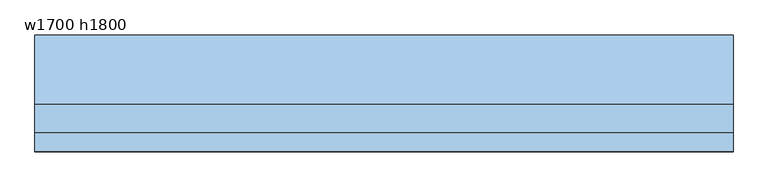
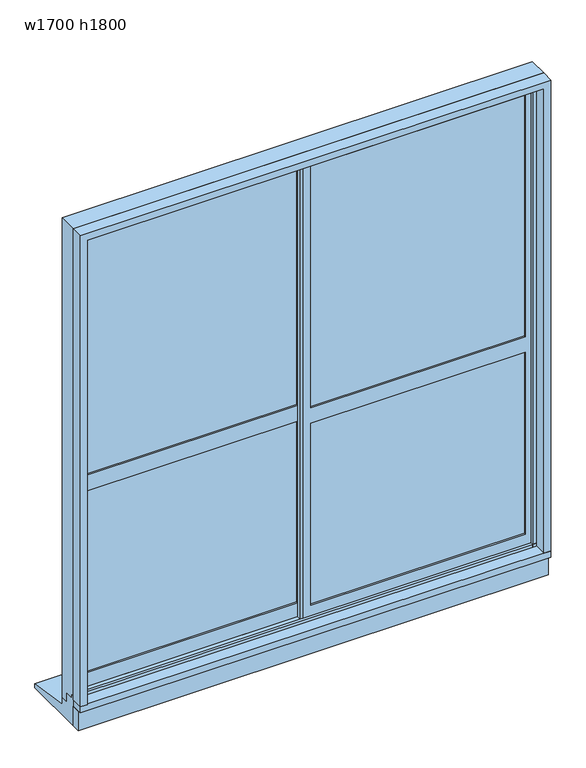
"""IFC4 building model written with IfcOpenShell, lengths in millimetres: window geometry, 引違い窓 2 枚 : w1700 h1800."""

from ifc_helpers import new_model, si_unit, frame, origin, place, context, project, spatial, polyline, outline, extrude, faceted_brep, source, transform, mapped, element, save


def w1700_h1800_203315db(model_context):
    return source(origin(), model_context, "Body", "SolidModel", [
        extrude(outline(polyline([(1860.0, -850.0), (60.0, -850.0), (60.0, -825.0), (1835.0, -825.0), (1835.0, 825.0), (60.0, 825.0), (60.0, 850.0), (1860.0, 850.0), (1860.0, -850.0)])), frame((0.0, -115.0, 0.0), z_axis=(0.0, 1.0, 0.0), x_axis=(0.0, 0.0, 1.0)), (0.0, 0.0, 1.0), 45.0),
        extrude(outline(polyline([(60.0, -850.0), (60.0, -825.0), (1835.0, -825.0), (1835.0, 825.0), (60.0, 825.0), (60.0, 850.0), (1860.0, 850.0), (1860.0, -850.0), (60.0, -850.0)])), frame((0.0, -115.0, 0.0), z_axis=(0.0, 1.0, 0.0), x_axis=(0.0, 0.0, 1.0)), (0.0, 0.0, 1.0), 45.0),
        extrude(outline(polyline([(850.0, -100.0), (-850.0, -100.0), (-850.0, -70.0), (850.0, -70.0), (850.0, -100.0)])), frame((0.0, 0.0, -40.0), z_axis=(0.0, 0.0, 1.0), x_axis=(1.0, 0.0, 0.0)), (0.0, 0.0, 1.0), 75.0),
        extrude(outline(polyline([(15.0, -28.0), (15.0, -42.0), (-15.0, -42.0), (-15.0, -28.0), (15.0, -28.0)])), frame((0.0, 0.0, 60.0), z_axis=(0.0, 0.0, 1.0), x_axis=(1.0, 0.0, 0.0)), (0.0, 0.0, 1.0), 1790.0),
        extrude(outline(polyline([(15.0, -48.5), (790.0, -48.5), (790.0, -53.5), (15.0, -53.5), (15.0, -48.5)])), frame((0.0, 0.0, 867.0), z_axis=(0.0, 0.0, 1.0), x_axis=(1.0, 0.0, 0.0)), (0.0, 0.0, 1.0), 923.0),
        extrude(outline(polyline([(15.0, -48.5), (790.0, -48.5), (790.0, -53.5), (15.0, -53.5), (15.0, -48.5)])), frame((0.0, 0.0, 113.0), z_axis=(0.0, 0.0, 1.0), x_axis=(1.0, 0.0, 0.0)), (0.0, 0.0, 1.0), 694.0),
        extrude(outline(polyline([(1850.0, -15.0), (60.0, -15.0), (60.0, 840.0), (1850.0, 840.0), (1850.0, -15.0)]), holes=[polyline([(807.0, 15.0), (807.0, 790.0), (113.0, 790.0), (113.0, 15.0), (807.0, 15.0)]), polyline([(867.0, 790.0), (867.0, 15.0), (1790.0, 15.0), (1790.0, 790.0), (867.0, 790.0)])]), frame((0.0, -60.0, 0.0), z_axis=(0.0, 1.0, 0.0), x_axis=(0.0, 0.0, 1.0)), (0.0, 0.0, 1.0), 18.0),
        extrude(outline(polyline([(-790.0, -16.5), (-15.0, -16.5), (-15.0, -21.5), (-790.0, -21.5), (-790.0, -16.5)])), frame((0.0, 0.0, 867.0), z_axis=(0.0, 0.0, 1.0), x_axis=(1.0, 0.0, 0.0)), (0.0, 0.0, 1.0), 923.0),
        extrude(outline(polyline([(-790.0, -16.5), (-15.0, -16.5), (-15.0, -21.5), (-790.0, -21.5), (-790.0, -16.5)])), frame((0.0, 0.0, 113.0), z_axis=(0.0, 0.0, 1.0), x_axis=(1.0, 0.0, 0.0)), (0.0, 0.0, 1.0), 694.0),
        extrude(outline(polyline([(1850.0, 15.0), (1850.0, -840.0), (60.0, -840.0), (60.0, 15.0), (1850.0, 15.0)]), holes=[polyline([(807.0, -15.0), (113.0, -15.0), (113.0, -790.0), (807.0, -790.0), (807.0, -15.0)]), polyline([(867.0, -790.0), (1790.0, -790.0), (1790.0, -15.0), (867.0, -15.0), (867.0, -790.0)])]), frame((0.0, -28.0, 0.0), z_axis=(0.0, 1.0, 0.0), x_axis=(0.0, 0.0, 1.0)), (0.0, 0.0, 1.0), 18.0),
        extrude(outline(polyline([(-70.0, -40.0), (-70.0, 73.0), (-60.0, 73.0), (-60.0, 60.0), (-28.0, 60.0), (-28.0, 26.0), (0.0, 26.0), (0.0, 0.0), (170.0, -25.0), (170.0, -40.0), (-70.0, -40.0)])), frame((-850.0, 0.0, 0.0), z_axis=(1.0, 0.0, 0.0), x_axis=(0.0, 1.0, 0.0)), (0.0, 0.0, 1.0), 1700.0),
        faceted_brep([(-850.0, -70.0, 26.0), (-850.0, 0.0, 26.0), (-810.0, 0.0, 26.0), (-810.0, -10.0, 26.0), (-840.0, -10.0, 26.0), (-840.0, -60.0, 26.0), (-810.0, -60.0, 26.0), (-810.0, -70.0, 26.0), (-850.0, -70.0, 1860.0), (-850.0, 0.0, 1860.0), (850.0, 0.0, 1860.0), (850.0, 0.0, 26.0), (810.0, 0.0, 26.0), (810.0, 0.0, 1820.0), (-810.0, 0.0, 1820.0), (-810.0, -10.0, 1820.0), (810.0, -10.0, 1820.0), (810.0, -10.0, 26.0), (840.0, -10.0, 26.0), (840.0, -10.0, 1850.0), (-840.0, -10.0, 1850.0), (-840.0, -60.0, 1850.0), (840.0, -60.0, 1850.0), (840.0, -60.0, 26.0), (810.0, -60.0, 26.0), (810.0, -60.0, 1820.0), (-810.0, -60.0, 1820.0), (-810.0, -70.0, 1820.0), (810.0, -70.0, 1820.0), (810.0, -70.0, 26.0), (850.0, -70.0, 26.0), (850.0, -70.0, 1860.0)], [[[0, 1, 2, 3, 4, 5, 6, 7]], [[1, 0, 8, 9]], [[2, 1, 9, 10, 11, 12, 13, 14]], [[3, 2, 14, 15]], [[4, 3, 15, 16, 17, 18, 19, 20]], [[5, 4, 20, 21]], [[6, 5, 21, 22, 23, 24, 25, 26]], [[7, 6, 26, 27]], [[0, 7, 27, 28, 29, 30, 31, 8]], [[9, 8, 31, 10]], [[15, 14, 13, 16]], [[21, 20, 19, 22]], [[27, 26, 25, 28]], [[30, 29, 24, 23, 18, 17, 12, 11]], [[10, 31, 30, 11]], [[16, 13, 12, 17]], [[22, 19, 18, 23]], [[28, 25, 24, 29]]]),
        extrude(outline(polyline([(-70.0, -40.0), (-70.0, 73.0), (-60.0, 73.0), (-60.0, 60.0), (-28.0, 60.0), (-28.0, 26.0), (0.0, 26.0), (0.0, 0.0), (170.0, -25.0), (170.0, -40.0), (-70.0, -40.0)])), frame((-850.0, 0.0, 0.0), z_axis=(1.0, 0.0, 0.0), x_axis=(0.0, 1.0, 0.0)), (0.0, 0.0, 1.0), 1700.0),
        extrude(outline(polyline([(-850.0, -70.0), (850.0, -70.0), (850.0, -115.0), (-850.0, -115.0), (-850.0, -70.0)])), frame((0.0, 0.0, 37.0), z_axis=(0.0, 0.0, 1.0), x_axis=(1.0, 0.0, 0.0)), (0.0, 0.0, 1.0), 25.0),
    ])


if __name__ == "__main__":
    model = new_model("IFC4")
    model_context = context("Model", 3, world=origin())
    ifc_project = project(units=[si_unit("LENGTHUNIT", "METRE", prefix="MILLI")], contexts=[model_context])
    site = spatial("IfcSite", under=ifc_project)
    building = spatial("IfcBuilding", under=site)
    placement = place(None, origin())
    w1700_h1800_shape = w1700_h1800_203315db(model_context)
    element("IfcWindow", 1, ObjectType="引違い窓 2 枚 : w1700 h1800", at=placement, inside=building, context=model_context, shape_type="MappedRepresentation", body=[
        mapped(w1700_h1800_shape, transform((0.0, 0.0, 0.0), x_axis=(1.0, 0.0, 0.0), y_axis=(0.0, 1.0, 0.0), z_axis=(0.0, 0.0, 1.0))),
    ])
    save(model, "model.ifc")

# Revit data of these elements
# Project information
#   プロジェクト発行日 = "発行日"
#   プロジェクト ステータス = "プロジェクト ステータス"
#   クライアント名 = "オーナ"
#   計画地住所 = "ここにアドレスを入力"
#   プロジェクト名 = "プロジェクト名"
#   プロジェクト番号 = "0001"
# Type "引違い窓 2 枚 : w1700 h1800"
#   Type Mark = "19"
#   Operation = "UserDefined"
#   Keynote = "08520.KK3"
#   Analytic Construction = "1/8 インチ ピルキントン一重ガラス"
#   Visual Light Transmittance = 0.9
#   Solar Heat Gain Coefficient = 0.78
#   Height = 1800 mm
#   Heat Transfer Coefficient (U) = 3.6886 W/(m²·K)
#   既定の腰高 = 60 mm
#   Width = 1700 mm
#   内枠見込み = 15 mm
#   サッシの幅 = 70 mm
#   内枠見附 = 25 mm
#   サッシ見附 = 40 mm
#   内枠 = 木目 - ナチュラル
#   内壁 = none
#   敷居 = 木目 - ナチュラル
#   サッシ = 金属 - アルミニウム
#   ガラス = ガラス - 透明
#   Wall Closure = (empty or 0)
# Element 1 (IfcWindow, "引違い窓 2 枚 : w1700 h1800")
#   Materials on its faces: "金属 - アルミニウム", "木目 - ナチュラル", "ガラス - 透明"
# Materials
#   "木目 - ナチュラル": class "木材", colour RGB 204 173 122, transparency 0
#   "金属 - アルミニウム": class "メタル", colour RGB 247 247 247, transparency 0
#   "ガラス - 透明": class "ガラス", colour RGB 0 128 255, transparency 0.9
